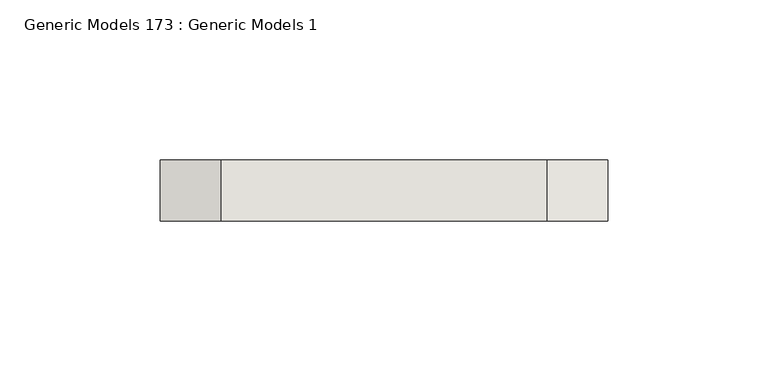
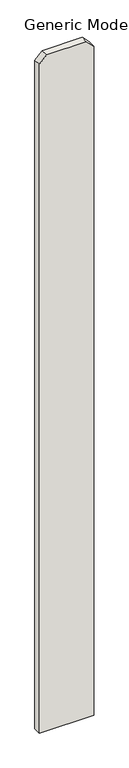
"""IFC4 building model written with IfcOpenShell, lengths in millimetres: wall geometry, Generic Models 173 : Generic Models 1."""

from ifc_helpers import new_model, si_unit, frame, origin, place, context, project, spatial, polyline, outline, extrude, source, transform, mapped, element, save


def generic_models_173_generic_models_1_6301b721(model_context):
    return source(origin(), model_context, "Body", "SweptSolid", [
        extrude(outline(polyline([(76.2, 325347.0125), (1885.95, 325347.0125), (1905.0, 325327.9625), (1905.0, 325226.3625), (1885.95, 325207.3125), (76.2, 325207.3125), (76.2, 325347.0125)])), frame((0.0, 547.6875, 0.0), z_axis=(0.0, 1.0, 0.0), x_axis=(0.0, 0.0, 1.0)), (0.0, 0.0, 1.0), 19.05),
    ])


if __name__ == "__main__":
    model = new_model("IFC4")
    model_context = context("Model", 3, world=origin())
    ifc_project = project(units=[si_unit("LENGTHUNIT", "METRE", prefix="MILLI")], contexts=[model_context])
    site = spatial("IfcSite", under=ifc_project)
    building = spatial("IfcBuilding", under=site)
    placement = place(None, origin())
    generic_models_173_generic_models_1_shape = generic_models_173_generic_models_1_6301b721(model_context)
    element("IfcWall", 1, ObjectType="Generic Models 173 : Generic Models 1", at=placement, inside=building, context=model_context, shape_type="MappedRepresentation", body=[
        mapped(generic_models_173_generic_models_1_shape, transform((0.0, 0.0, 0.0), x_axis=(1.0, 0.0, 0.0), y_axis=(0.0, 1.0, 0.0), z_axis=(0.0, 0.0, 1.0))),
    ])
    save(model, "model.ifc")

# Revit data of these elements
# Element 1 (IfcWall, "Generic Models 173 : Generic Models 1")
#   Materials on its faces: "VERTICAL 1X6 CEDAR PLANKS W/ CLEAR WOOD SEALER"
# Materials
#   "VERTICAL 1X6 CEDAR PLANKS W/ CLEAR WOOD SEALER": class "Wood", colour RGB 234 198 147, transparency 0, Description = "Pinus Echinata", Cost = 0
